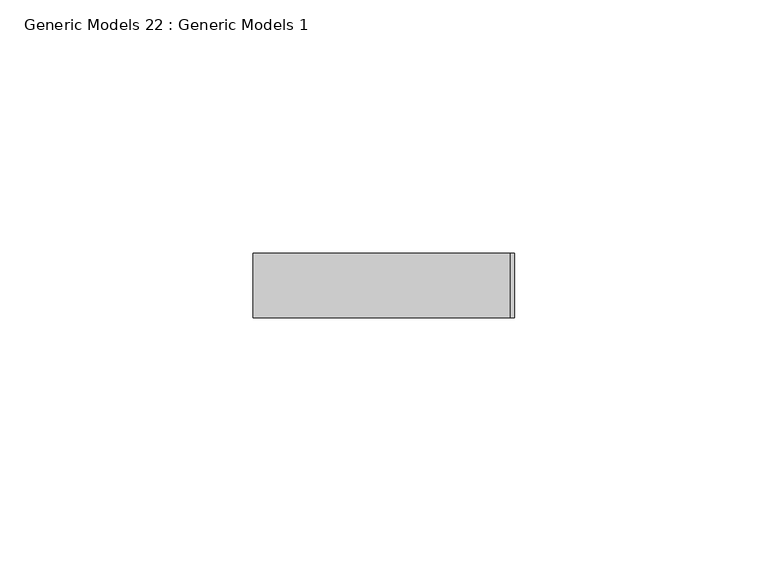
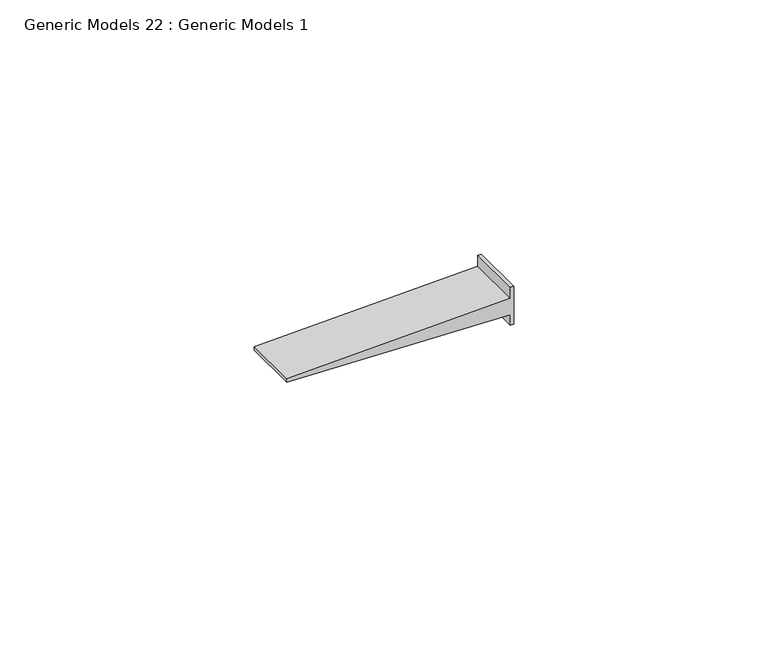
"""IFC4 building model written with IfcOpenShell, lengths in millimetres: proxy geometry, Generic Models 22 : Generic Models 1."""

import ifcopenshell
import ifcopenshell.guid

model = None  # the IFC model being written
_history = None  # IfcOwnerHistory: only IFC2X3 demands one
_inside = {}  # id of a spatial element -> (the spatial element, [elements in it])
_under = {}  # id of a project, library or spatial element -> (it, [spatial elements below it])
_declared = {}  # id of a project -> (the project, [libraries it declares])
_typed = {}  # id of a type object -> (the type object, [elements of that type])
_made_of = {}  # id of a material, layer set ... -> (it, [elements and type objects made of it])


def new_model(schema):
    """Start an empty IFC model of exactly this schema.

    Asked for "IFC4X3", IfcOpenShell would pick the latest addendum, in which some entities
    have other attributes; the version numbers below select the first issue.
    IFC2X3 requires an IfcOwnerHistory on every rooted entity: one is made here for all.
    """
    global model, _history
    if schema == "IFC4X3":
        model = ifcopenshell.file(schema_version=(4, 3, 0, 0))
    else:
        model = ifcopenshell.file(schema=schema)
    _inside.clear()
    _under.clear()
    _declared.clear()
    _typed.clear()
    _made_of.clear()
    _history = None
    if model.schema == "IFC2X3":
        org = make("IfcOrganization", Name="unknown")
        user = make(
            "IfcPersonAndOrganization",
            ThePerson=make("IfcPerson", FamilyName="unknown"),
            TheOrganization=org,
        )
        app = make(
            "IfcApplication",
            ApplicationDeveloper=org,
            Version="unknown",
            ApplicationFullName="unknown",
            ApplicationIdentifier="unknown",
        )
        _history = make(
            "IfcOwnerHistory",
            OwningUser=user,
            OwningApplication=app,
            ChangeAction="ADDED",
            CreationDate=0,
        )
    return model


def make(cls, **values):
    """One entity of the class cls with the attributes given. An attribute that is None is left unset."""
    return model.create_entity(
        cls, **{name: value for name, value in values.items() if value is not None}
    )


def rooted(cls, **values):
    """An entity with a GlobalId (a new one), such as an element, a storey or a relation."""
    return make(cls, GlobalId=ifcopenshell.guid.new(), OwnerHistory=_history, **values)


def si_unit(unit_type, name, prefix=None):
    """IfcSIUnit, for example si_unit("LENGTHUNIT", "METRE", prefix="MILLI")."""
    return make("IfcSIUnit", UnitType=unit_type, Prefix=prefix, Name=name)


def assignment(units):
    """IfcUnitAssignment: the units of a project."""
    return None if units is None else make("IfcUnitAssignment", Units=units)


def point(xyz):
    """IfcCartesianPoint."""
    return None if xyz is None else make("IfcCartesianPoint", Coordinates=xyz)


def direction(xyz):
    """IfcDirection."""
    return None if xyz is None else make("IfcDirection", DirectionRatios=xyz)


def frame(location, z_axis=None, x_axis=None):
    """IfcAxis2Placement3D, a coordinate frame: its origin and axes. An axis left out is left unset."""
    return make(
        "IfcAxis2Placement3D",
        Location=point(location),
        Axis=direction(z_axis),
        RefDirection=direction(x_axis),
    )


def origin():
    """The frame at (0, 0, 0) with its axes left unset."""
    return frame((0.0, 0.0, 0.0))


def place(relative_to, where):
    """IfcLocalPlacement: puts the frame where relative to a parent placement (None: the world)."""
    return make(
        "IfcLocalPlacement", PlacementRelTo=relative_to, RelativePlacement=where
    )


def context(
    kind, dimensions, precision=None, world=None, true_north=None, identifier=None
):
    """IfcGeometricRepresentationContext, for example the 3D "Model" context."""
    return make(
        "IfcGeometricRepresentationContext",
        ContextIdentifier=identifier,
        ContextType=kind,
        CoordinateSpaceDimension=dimensions,
        Precision=precision,
        WorldCoordinateSystem=world,
        TrueNorth=true_north,
    )


def project(units=None, contexts=None):
    """IfcProject with its units and contexts."""
    return rooted(
        "IfcProject",
        Name="project",
        RepresentationContexts=contexts,
        UnitsInContext=assignment(units),
    )


def spatial(cls, under=None, at=None, **own):
    """A site, building, storey or space (cls), placed at a placement, below another one or the project."""
    s = rooted(cls, ObjectPlacement=at, **own)
    if under is not None:
        _under.setdefault(under.id(), (under, []))[1].append(s)
    return s


def polyline(points):
    """IfcPolyline through the points."""
    return make("IfcPolyline", Points=[point(p) for p in points])


def outline(outer, holes=None, kind="AREA"):
    """IfcArbitraryClosedProfileDef: a profile drawn as a closed curve; with holes, ...WithVoids."""
    if holes is None:
        return make("IfcArbitraryClosedProfileDef", ProfileType=kind, OuterCurve=outer)
    return make(
        "IfcArbitraryProfileDefWithVoids",
        ProfileType=kind,
        OuterCurve=outer,
        InnerCurves=holes,
    )


def extrude(swept, where, along, depth):
    """IfcExtrudedAreaSolid: the profile swept, set in the frame where, extruded along a direction by depth."""
    return make(
        "IfcExtrudedAreaSolid",
        SweptArea=swept,
        Position=where,
        ExtrudedDirection=direction(along),
        Depth=depth,
    )


def shape(context_of_items, identifier, shape_type, items):
    """IfcShapeRepresentation: the items that make up one representation, for example the "Body"."""
    return make(
        "IfcShapeRepresentation",
        ContextOfItems=context_of_items,
        RepresentationIdentifier=identifier,
        RepresentationType=shape_type,
        Items=items,
    )


def source(mapping_origin, context_of_items, identifier, shape_type, items):
    """IfcRepresentationMap: a shape defined once, which mapped items show again and again."""
    return make(
        "IfcRepresentationMap",
        MappingOrigin=mapping_origin,
        MappedRepresentation=shape(context_of_items, identifier, shape_type, items),
    )


def transform(
    local_origin,
    x_axis=None,
    y_axis=None,
    z_axis=None,
    scale=None,
    scale2=None,
    scale3=None,
    uniform=True,
):
    """IfcCartesianTransformationOperator3D, or its non-uniform kind. x_axis, y_axis, z_axis: its Axis1, 2, 3."""
    if uniform:
        return make(
            "IfcCartesianTransformationOperator3D",
            Axis1=direction(x_axis),
            Axis2=direction(y_axis),
            LocalOrigin=point(local_origin),
            Scale=scale,
            Axis3=direction(z_axis),
        )
    return make(
        "IfcCartesianTransformationOperator3DnonUniform",
        Axis1=direction(x_axis),
        Axis2=direction(y_axis),
        LocalOrigin=point(local_origin),
        Scale=scale,
        Axis3=direction(z_axis),
        Scale2=scale2,
        Scale3=scale3,
    )


def mapped(mapping_source, mapping_target):
    """IfcMappedItem: shows the shape of a source again, moved by a transform."""
    return make(
        "IfcMappedItem", MappingSource=mapping_source, MappingTarget=mapping_target
    )


def made_of(thing, what):
    """Note that an element or type object is made of a material, layer set ...; save() writes the relation."""
    if what is not None:
        _made_of.setdefault(what.id(), (what, []))[1].append(thing)
    return thing


def element(
    cls,
    number,
    at=None,
    inside=None,
    cuts=None,
    type_object=None,
    material=None,
    context=None,
    identifier="Body",
    shape_type=None,
    held_by="IfcProductDefinitionShape",
    body=None,
    shapes=None,
    **own,
):
    """One element of the class cls, such as IfcWall. Its Tag is "e" and its number.

    at: its placement. inside: the storey or other place that contains it. cuts: it is an
    opening in that element (IfcRelVoidsElement). A single representation is given by context,
    identifier, shape_type and body (its items); several are given by shapes. held_by: the class
    of the entity that holds the representations. save() writes the other relations.
    """
    e = rooted(cls, Tag="e%d" % number, ObjectPlacement=at, **own)
    if body is not None:
        shapes = [shape(context, identifier, shape_type, body)]
    if shapes is not None:
        e.Representation = make(held_by, Representations=shapes)
    if inside is not None:
        _inside.setdefault(inside.id(), (inside, []))[1].append(e)
    if cuts is not None:
        rooted(
            "IfcRelVoidsElement", RelatingBuildingElement=cuts, RelatedOpeningElement=e
        )
    if type_object is not None:
        _typed.setdefault(type_object.id(), (type_object, []))[1].append(e)
    return made_of(e, material)


def aggregate(whole, parts):
    """IfcRelAggregates: a whole, such as a stair, and the parts it consists of."""
    return rooted("IfcRelAggregates", RelatingObject=whole, RelatedObjects=parts)


def save(model, path):
    """Write the relations noted so far, then the file.

    IfcRelAggregates (storeys below a building ...), IfcRelContainedInSpatialStructure (elements
    in a storey), IfcRelDefinesByType, IfcRelAssociatesMaterial and IfcRelDeclares: one each for
    every whole, place, type object, material and project.
    """
    for whole, parts in _under.values():
        aggregate(whole, parts)
    for where, things in _inside.values():
        rooted(
            "IfcRelContainedInSpatialStructure",
            RelatedElements=things,
            RelatingStructure=where,
        )
    for kind, things in _typed.values():
        rooted("IfcRelDefinesByType", RelatedObjects=things, RelatingType=kind)
    for what, things in _made_of.values():
        rooted("IfcRelAssociatesMaterial", RelatedObjects=things, RelatingMaterial=what)
    for by, libraries in _declared.values():
        rooted("IfcRelDeclares", RelatingContext=by, RelatedDefinitions=libraries)
    model.write(path)


def generic_models_22_generic_models_1_e5767157(model_context):
    return source(origin(), model_context, "Body", "SweptSolid", [
        extrude(outline(polyline([(2409.6091, 49800.66875), (2409.6091, 49799.875), (2407.0592364, 49799.875), (2405.4618473, 49749.075), (2404.6631527, 49749.075), (2403.0657636, 49799.875), (2400.5159, 49799.875), (2400.5159, 49800.66875), (2409.6091, 49800.66875)])), frame((0.0, 565.15, 0.0), z_axis=(0.0, 1.0, 0.0), x_axis=(0.0, 0.0, 1.0)), (0.0, 0.0, 1.0), 12.7),
    ])


if __name__ == "__main__":
    model = new_model("IFC4")
    model_context = context("Model", 3, world=origin())
    ifc_project = project(units=[si_unit("LENGTHUNIT", "METRE", prefix="MILLI")], contexts=[model_context])
    site = spatial("IfcSite", under=ifc_project)
    building = spatial("IfcBuilding", under=site)
    placement = place(None, origin())
    generic_models_22_generic_models_1_shape = generic_models_22_generic_models_1_e5767157(model_context)
    element("IfcBuildingElementProxy", 1, Name="Generic Models 22 : Generic Models 1", ObjectType="Generic Models 22 : Generic Models 1", at=placement, inside=building, context=model_context, shape_type="MappedRepresentation", body=[
        mapped(generic_models_22_generic_models_1_shape, transform((0.0, 0.0, 0.0), x_axis=(1.0, 0.0, 0.0), y_axis=(0.0, 1.0, 0.0), z_axis=(0.0, 0.0, 1.0))),
    ])
    save(model, "model.ifc")

# Revit data of these elements
# Element 1 (IfcBuildingElementProxy, "Generic Models 22 : Generic Models 1")
#   Materials on its faces: "ATTACH GYPSUM BOARD TO STUDS AND NOT TO TOP TRACK"
# Materials
#   "ATTACH GYPSUM BOARD TO STUDS AND NOT TO TOP TRACK": class "Generic", colour RGB 48 48 48, transparency 0, Cost = 0
